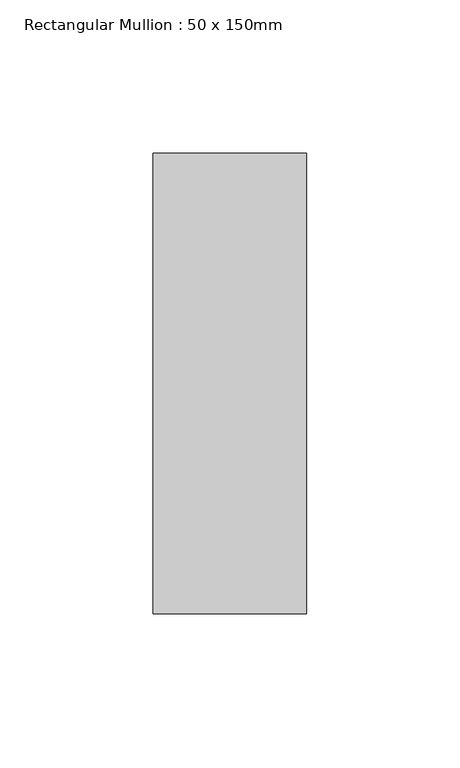
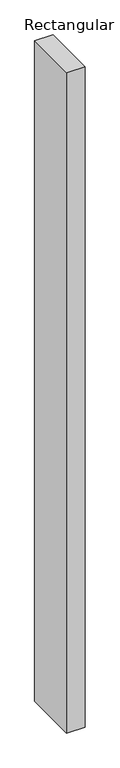
"""IFC4 building model written with IfcOpenShell, lengths in millimetres: member geometry, Rectangular Mullion : 50 x 150mm."""

from ifc_helpers import new_model, si_unit, frame, origin, place, context, project, spatial, polyline, outline, extrude, source, transform, mapped, element, save


def rectangular_mullion_50_x_150mm_e9a32396(model_context):
    return source(origin(), model_context, "Body", "SweptSolid", [
        extrude(outline(polyline([(0.0, 75.0), (0.0, -75.0), (-50.0, -75.0), (-50.0, 75.0), (0.0, 75.0)])), frame((0.0, 0.0, -1899.9999997), z_axis=(0.0, 0.0, 1.0), x_axis=(1.0, 0.0, 0.0)), (0.0, 0.0, 1.0), 1899.9999997),
    ])


if __name__ == "__main__":
    model = new_model("IFC4")
    model_context = context("Model", 3, world=origin())
    ifc_project = project(units=[si_unit("LENGTHUNIT", "METRE", prefix="MILLI")], contexts=[model_context])
    site = spatial("IfcSite", under=ifc_project)
    building = spatial("IfcBuilding", under=site)
    placement = place(None, origin())
    rectangular_mullion_50_x_150mm_shape = rectangular_mullion_50_x_150mm_e9a32396(model_context)
    element("IfcMember", 1, ObjectType="Rectangular Mullion : 50 x 150mm", at=placement, inside=building, context=model_context, shape_type="MappedRepresentation", body=[
        mapped(rectangular_mullion_50_x_150mm_shape, transform((0.0, 0.0, 0.0), x_axis=(1.0, 0.0, 0.0), y_axis=(0.0, 1.0, 0.0), z_axis=(0.0, 0.0, 1.0))),
    ])
    save(model, "model.ifc")

# Revit data of these elements
# Type "Rectangular Mullion : 50 x 150mm"
#   built-in parameter 1007304 = 0.492126 (stored number, unit not read)
#   built-in parameter 1007301 = 0.082021 (stored number, unit not read)
#   built-in parameter 1007300 = 0.082021 (stored number, unit not read)
# Element 1 (IfcMember, "Rectangular Mullion : 50 x 150mm")
#   Materials on its faces: "Metal - Aluminium"
# Materials
#   "Metal - Aluminium": class "Metal", colour RGB 247 247 247, transparency 0
